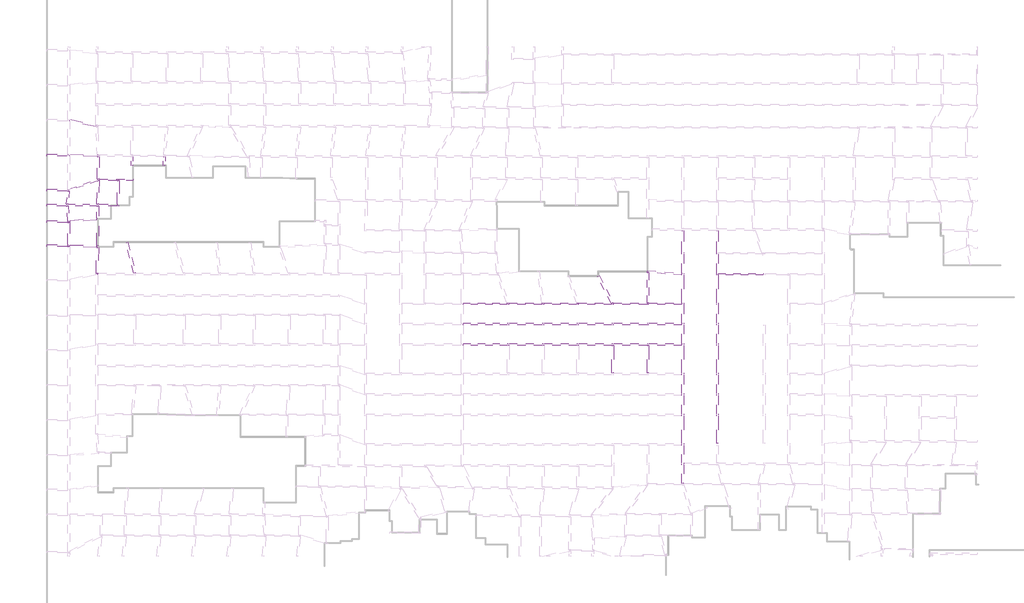
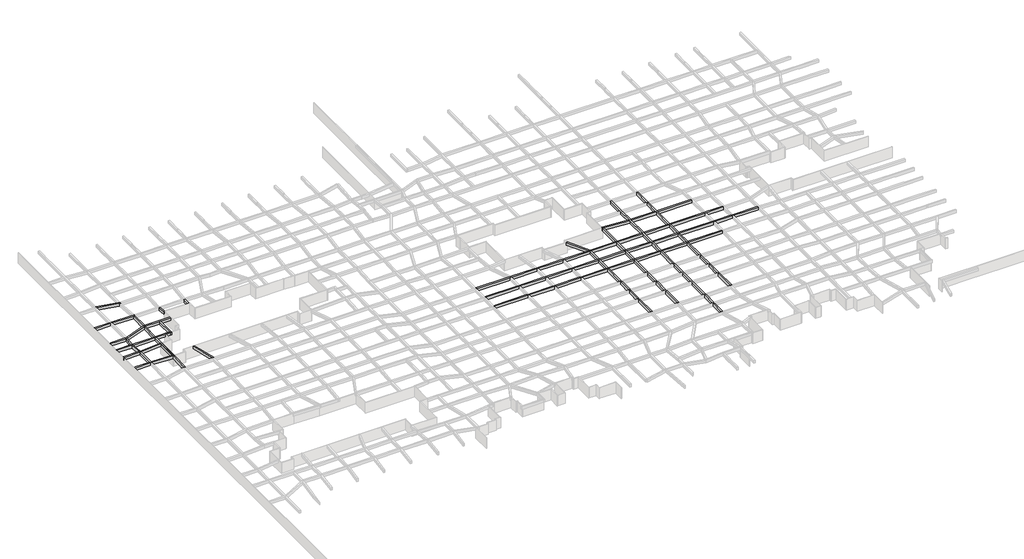
# One storey, part 34 of 45: 33 beams.
"""IFC4 building model written with IfcOpenShell, lengths in millimetres."""

import ifcopenshell
import ifcopenshell.guid

model = None  # the IFC model being written
_history = None  # IfcOwnerHistory: only IFC2X3 demands one
_inside = {}  # id of a spatial element -> (the spatial element, [elements in it])
_under = {}  # id of a project, library or spatial element -> (it, [spatial elements below it])
_declared = {}  # id of a project -> (the project, [libraries it declares])
_typed = {}  # id of a type object -> (the type object, [elements of that type])
_made_of = {}  # id of a material, layer set ... -> (it, [elements and type objects made of it])


def new_model(schema):
    """Start an empty IFC model of exactly this schema.

    Asked for "IFC4X3", IfcOpenShell would pick the latest addendum, in which some entities
    have other attributes; the version numbers below select the first issue.
    IFC2X3 requires an IfcOwnerHistory on every rooted entity: one is made here for all.
    """
    global model, _history
    if schema == "IFC4X3":
        model = ifcopenshell.file(schema_version=(4, 3, 0, 0))
    else:
        model = ifcopenshell.file(schema=schema)
    _inside.clear()
    _under.clear()
    _declared.clear()
    _typed.clear()
    _made_of.clear()
    _history = None
    if model.schema == "IFC2X3":
        org = make("IfcOrganization", Name="unknown")
        user = make(
            "IfcPersonAndOrganization",
            ThePerson=make("IfcPerson", FamilyName="unknown"),
            TheOrganization=org,
        )
        app = make(
            "IfcApplication",
            ApplicationDeveloper=org,
            Version="unknown",
            ApplicationFullName="unknown",
            ApplicationIdentifier="unknown",
        )
        _history = make(
            "IfcOwnerHistory",
            OwningUser=user,
            OwningApplication=app,
            ChangeAction="ADDED",
            CreationDate=0,
        )
    return model


def make(cls, **values):
    """One entity of the class cls with the attributes given. An attribute that is None is left unset."""
    return model.create_entity(
        cls, **{name: value for name, value in values.items() if value is not None}
    )


def rooted(cls, **values):
    """An entity with a GlobalId (a new one), such as an element, a storey or a relation."""
    return make(cls, GlobalId=ifcopenshell.guid.new(), OwnerHistory=_history, **values)


def si_unit(unit_type, name, prefix=None):
    """IfcSIUnit, for example si_unit("LENGTHUNIT", "METRE", prefix="MILLI")."""
    return make("IfcSIUnit", UnitType=unit_type, Prefix=prefix, Name=name)


def assignment(units):
    """IfcUnitAssignment: the units of a project."""
    return None if units is None else make("IfcUnitAssignment", Units=units)


def point(xyz):
    """IfcCartesianPoint."""
    return None if xyz is None else make("IfcCartesianPoint", Coordinates=xyz)


def direction(xyz):
    """IfcDirection."""
    return None if xyz is None else make("IfcDirection", DirectionRatios=xyz)


def frame(location, z_axis=None, x_axis=None):
    """IfcAxis2Placement3D, a coordinate frame: its origin and axes. An axis left out is left unset."""
    return make(
        "IfcAxis2Placement3D",
        Location=point(location),
        Axis=direction(z_axis),
        RefDirection=direction(x_axis),
    )


def origin():
    """The frame at (0, 0, 0) with its axes left unset."""
    return frame((0.0, 0.0, 0.0))


def place(relative_to, where):
    """IfcLocalPlacement: puts the frame where relative to a parent placement (None: the world)."""
    return make(
        "IfcLocalPlacement", PlacementRelTo=relative_to, RelativePlacement=where
    )


def context(
    kind, dimensions, precision=None, world=None, true_north=None, identifier=None
):
    """IfcGeometricRepresentationContext, for example the 3D "Model" context."""
    return make(
        "IfcGeometricRepresentationContext",
        ContextIdentifier=identifier,
        ContextType=kind,
        CoordinateSpaceDimension=dimensions,
        Precision=precision,
        WorldCoordinateSystem=world,
        TrueNorth=true_north,
    )


def project(units=None, contexts=None):
    """IfcProject with its units and contexts."""
    return rooted(
        "IfcProject",
        Name="project",
        RepresentationContexts=contexts,
        UnitsInContext=assignment(units),
    )


def spatial(cls, under=None, at=None, **own):
    """A site, building, storey or space (cls), placed at a placement, below another one or the project."""
    s = rooted(cls, ObjectPlacement=at, **own)
    if under is not None:
        _under.setdefault(under.id(), (under, []))[1].append(s)
    return s


def polyline(points):
    """IfcPolyline through the points."""
    return make("IfcPolyline", Points=[point(p) for p in points])


def outline(outer, holes=None, kind="AREA"):
    """IfcArbitraryClosedProfileDef: a profile drawn as a closed curve; with holes, ...WithVoids."""
    if holes is None:
        return make("IfcArbitraryClosedProfileDef", ProfileType=kind, OuterCurve=outer)
    return make(
        "IfcArbitraryProfileDefWithVoids",
        ProfileType=kind,
        OuterCurve=outer,
        InnerCurves=holes,
    )


def extrude(swept, where, along, depth):
    """IfcExtrudedAreaSolid: the profile swept, set in the frame where, extruded along a direction by depth."""
    return make(
        "IfcExtrudedAreaSolid",
        SweptArea=swept,
        Position=where,
        ExtrudedDirection=direction(along),
        Depth=depth,
    )


def faces_of(points, faces, orient=None, outer=None):
    """IfcFace entities. A face is a list of loops; a loop is a list of indices into points, from 0.

    orient and outer hold one flag for each loop. By default every Orientation is true, the
    first loop of a face is its IfcFaceOuterBound and the others are IfcFaceBound.
    """
    made = []
    for i, loops in enumerate(faces):
        bounds = []
        for j, loop in enumerate(loops):
            is_outer = j == 0 if outer is None else outer[i][j]
            bounds.append(
                make(
                    "IfcFaceOuterBound" if is_outer else "IfcFaceBound",
                    Bound=make("IfcPolyLoop", Polygon=[points[k] for k in loop]),
                    Orientation=True if orient is None else orient[i][j],
                )
            )
        made.append(make("IfcFace", Bounds=bounds))
    return made


def faceted_brep(points, faces, orient=None, outer=None, voids=None):
    """IfcFacetedBrep: a solid bounded by flat faces; with voids (closed shells), ...WithVoids."""
    shared = [point(p) for p in points]
    hull = make("IfcClosedShell", CfsFaces=faces_of(shared, faces, orient, outer))
    if voids is None:
        return make("IfcFacetedBrep", Outer=hull)
    return make(
        "IfcFacetedBrepWithVoids",
        Outer=hull,
        Voids=[
            make(cls, CfsFaces=faces_of(shared, fs, o, b)) for cls, fs, o, b in voids
        ],
    )


def shape(context_of_items, identifier, shape_type, items):
    """IfcShapeRepresentation: the items that make up one representation, for example the "Body"."""
    return make(
        "IfcShapeRepresentation",
        ContextOfItems=context_of_items,
        RepresentationIdentifier=identifier,
        RepresentationType=shape_type,
        Items=items,
    )


def made_of(thing, what):
    """Note that an element or type object is made of a material, layer set ...; save() writes the relation."""
    if what is not None:
        _made_of.setdefault(what.id(), (what, []))[1].append(thing)
    return thing


def element(
    cls,
    number,
    at=None,
    inside=None,
    cuts=None,
    type_object=None,
    material=None,
    context=None,
    identifier="Body",
    shape_type=None,
    held_by="IfcProductDefinitionShape",
    body=None,
    shapes=None,
    **own,
):
    """One element of the class cls, such as IfcWall. Its Tag is "e" and its number.

    at: its placement. inside: the storey or other place that contains it. cuts: it is an
    opening in that element (IfcRelVoidsElement). A single representation is given by context,
    identifier, shape_type and body (its items); several are given by shapes. held_by: the class
    of the entity that holds the representations. save() writes the other relations.
    """
    e = rooted(cls, Tag="e%d" % number, ObjectPlacement=at, **own)
    if body is not None:
        shapes = [shape(context, identifier, shape_type, body)]
    if shapes is not None:
        e.Representation = make(held_by, Representations=shapes)
    if inside is not None:
        _inside.setdefault(inside.id(), (inside, []))[1].append(e)
    if cuts is not None:
        rooted(
            "IfcRelVoidsElement", RelatingBuildingElement=cuts, RelatedOpeningElement=e
        )
    if type_object is not None:
        _typed.setdefault(type_object.id(), (type_object, []))[1].append(e)
    return made_of(e, material)


def aggregate(whole, parts):
    """IfcRelAggregates: a whole, such as a stair, and the parts it consists of."""
    return rooted("IfcRelAggregates", RelatingObject=whole, RelatedObjects=parts)


def save(model, path):
    """Write the relations noted so far, then the file.

    IfcRelAggregates (storeys below a building ...), IfcRelContainedInSpatialStructure (elements
    in a storey), IfcRelDefinesByType, IfcRelAssociatesMaterial and IfcRelDeclares: one each for
    every whole, place, type object, material and project.
    """
    for whole, parts in _under.values():
        aggregate(whole, parts)
    for where, things in _inside.values():
        rooted(
            "IfcRelContainedInSpatialStructure",
            RelatedElements=things,
            RelatingStructure=where,
        )
    for kind, things in _typed.values():
        rooted("IfcRelDefinesByType", RelatedObjects=things, RelatingType=kind)
    for what, things in _made_of.values():
        rooted("IfcRelAssociatesMaterial", RelatedObjects=things, RelatingMaterial=what)
    for by, libraries in _declared.values():
        rooted("IfcRelDeclares", RelatingContext=by, RelatedDefinitions=libraries)
    model.write(path)


model = new_model("IFC4")

# Units and contexts
model_context = context("Model", 3, world=origin())
ifc_project = project(units=[si_unit("LENGTHUNIT", "METRE", prefix="MILLI")], contexts=[model_context])

# Site, building, storey
site = spatial("IfcSite", under=ifc_project)
building = spatial("IfcBuilding", under=site)
storey = spatial("IfcBuildingStorey", under=building, Name="户型图", Elevation=0.0)

# Beams
placement = place(None, origin())
element("IfcBeam", 1, ObjectType="混凝土 - 矩形梁 : KL_beam", at=placement, inside=storey, context=model_context, shape_type="Brep", body=[
    faceted_brep([(-143382.0266166, 146959.1608501, 3300.0), (-143382.0266166, 147100.0740901, 3300.0), (-143382.0266166, 147301.8194636, 3300.0), (-143382.0266166, 147382.2091225, 3300.0), (-143782.0266166, 147244.4780772, 3300.0), (-149980.0650049, 145110.3223119, 3300.0), (-149980.0650049, 144687.2740394, 3300.0), (-143786.9810795, 146819.7238463, 3300.0), (-143384.5011388, 146958.3088037, 3300.0), (-143382.0266166, 146959.1608501, 2500.0), (-149980.0650049, 144687.2740394, 2500.0), (-143786.9810795, 146819.7238463, 2500.0), (-143384.5011388, 146958.3088037, 2500.0), (-143382.0266166, 147382.2091225, 2500.0), (-143382.0266166, 147301.8194636, 2500.0), (-143382.0266166, 147100.0740901, 2500.0), (-149980.0650049, 145110.3223119, 2500.0), (-143782.0266166, 147244.4780772, 2500.0)], [[[0, 1, 2, 3, 4, 5, 6, 7, 8]], [[9, 0, 8, 7, 6, 10, 11, 12]], [[13, 14, 15, 9, 12, 11, 10, 16, 17]], [[3, 13, 17, 16, 5, 4]], [[6, 5, 16, 10]], [[3, 2, 1, 0, 9, 15, 14, 13]]]),
])
element("IfcBeam", 2, ObjectType="混凝土 - 矩形梁 : KL_beam", at=placement, inside=storey, context=model_context, shape_type="SweptSolid", body=[
    extrude(outline(polyline([(-155040.2933307, 152429.932653), (-155040.2933307, 152829.932653), (-150380.0650049, 152829.932653), (-150380.0650049, 152429.932653), (-155040.2933307, 152429.932653)])), frame((0.0, 0.0, 2500.0), z_axis=(0.0, 0.0, 1.0), x_axis=(1.0, 0.0, 0.0)), (0.0, 0.0, 1.0), 800.0),
])
element("IfcBeam", 3, ObjectType="混凝土 - 矩形梁 : KL_beam", at=placement, inside=storey, context=model_context, shape_type="Brep", body=[
    faceted_brep([(-155040.2933307, 145029.932653, 3300.0), (-155040.2933307, 145029.932653, 2500.0), (-155040.2933307, 144629.932653, 2500.0), (-155040.2933307, 144629.932653, 3300.0), (-150398.2249808, 144629.932653, 3300.0), (-150146.5964831, 144629.932653, 3300.0), (-149992.0411016, 144683.1503386, 3300.0), (-149980.0650049, 144687.2740394, 3300.0), (-150380.0650049, 144687.2740394, 3300.0), (-150380.0650049, 144972.5912666, 3300.0), (-150380.0650049, 145029.932653, 3300.0), (-150398.2249808, 144629.932653, 2500.0), (-150146.5964831, 144629.932653, 2500.0), (-150380.0650049, 145029.932653, 2500.0), (-150380.0650049, 144972.5912666, 2500.0), (-150380.0650049, 144687.2740394, 2500.0), (-149980.0650049, 144687.2740394, 2500.0), (-149992.0411016, 144683.1503386, 2500.0)], [[[0, 1, 2, 3]], [[0, 3, 4, 5, 6, 7, 8, 9, 10]], [[3, 2, 11, 12, 5, 4]], [[2, 1, 13, 14, 15, 16, 17, 12, 11]], [[1, 0, 10, 13]], [[7, 6, 5, 12, 17, 16]], [[8, 15, 14, 13, 10, 9]], [[15, 8, 7, 16]]]),
])
element("IfcBeam", 4, ObjectType="混凝土 - 矩形梁 : KL_beam", at=placement, inside=storey, context=model_context, shape_type="Brep", body=[
    faceted_brep([(-143707.512981, 158849.6325984, 3300.0), (-143710.0525927, 158899.3775215, 3300.0), (-143728.6193094, 159263.055125, 3300.0), (-143899.5027499, 159299.3775215, 3300.0), (-144130.8224936, 159348.5460509, 3300.0), (-149980.0650049, 160591.8409275, 3300.0), (-149980.0650049, 160182.9046895, 3300.0), (-144112.4278844, 158935.6999181, 3300.0), (-143707.512981, 158849.6325984, 2500.0), (-149980.0650049, 160182.9046895, 2500.0), (-144112.4278844, 158935.6999181, 2500.0), (-143728.6193094, 159263.055125, 2500.0), (-143710.0525927, 158899.3775215, 2500.0), (-149980.0650049, 160591.8409275, 2500.0), (-144130.8224936, 159348.5460509, 2500.0), (-143899.5027499, 159299.3775215, 2500.0)], [[[0, 1, 2, 3, 4, 5, 6, 7]], [[8, 0, 7, 6, 9, 10]], [[11, 12, 8, 10, 9, 13, 14, 15]], [[2, 11, 15, 14, 13, 5, 4, 3]], [[6, 5, 13, 9]], [[2, 1, 0, 8, 12, 11]]]),
])
element("IfcBeam", 5, ObjectType="混凝土 - 矩形梁 : KL_beam", at=placement, inside=storey, context=model_context, shape_type="Brep", body=[
    faceted_brep([(-143401.4944506, 152264.5687631, 3300.0), (-143391.7428195, 152664.4498776, 3300.0), (-143792.7630206, 152674.2292868, 3300.0), (-149980.0650049, 152825.1148483, 3300.0), (-149980.0650049, 152424.9959274, 3300.0), (-143782.0266166, 152273.8485445, 3300.0), (-143401.4944506, 152264.5687631, 2500.0), (-149980.0650049, 152424.9959274, 2500.0), (-143782.0266166, 152273.8485445, 2500.0), (-143391.7428195, 152664.4498776, 2500.0), (-149980.0650049, 152825.1148483, 2500.0), (-143792.7630206, 152674.2292868, 2500.0)], [[[0, 1, 2, 3, 4, 5]], [[6, 0, 5, 4, 7, 8]], [[9, 6, 8, 7, 10, 11]], [[1, 9, 11, 10, 3, 2]], [[4, 3, 10, 7]], [[1, 0, 6, 9]]]),
])
element("IfcBeam", 6, ObjectType="混凝土 - 矩形梁 : KL_beam", at=placement, inside=storey, context=model_context, shape_type="Brep", body=[
    faceted_brep([(-143382.0266166, 147382.2091225, 3300.0), (-143382.0266166, 152269.0307398, 3300.0), (-143382.0266166, 152664.2129351, 3300.0), (-143391.7428195, 152664.4498776, 3300.0), (-143401.4944506, 152264.5687631, 3300.0), (-143772.3104136, 152273.611602, 3300.0), (-143782.0266166, 152273.8485445, 3300.0), (-143782.0266166, 147244.4780772, 3300.0), (-143782.0266166, 147244.4780772, 2500.0), (-143782.0266166, 152273.8485445, 2500.0), (-143382.0266166, 152664.2129351, 2500.0), (-143382.0266166, 152269.0307398, 2500.0), (-143382.0266166, 147382.2091225, 2500.0), (-143772.3104136, 152273.611602, 2500.0), (-143401.4944506, 152264.5687631, 2500.0), (-143391.7428195, 152664.4498776, 2500.0)], [[[0, 1, 2, 3, 4, 5, 6, 7]], [[8, 7, 6, 9]], [[10, 11, 12, 8, 9, 13, 14, 15]], [[2, 1, 0, 12, 11, 10]], [[15, 3, 2, 10]], [[0, 7, 8, 12]], [[4, 14, 13, 9, 6, 5]], [[14, 4, 3, 15]]]),
])
element("IfcBeam", 7, ObjectType="混凝土 - 矩形梁 : KL_beam", at=placement, inside=storey, context=model_context, shape_type="Brep", body=[
    faceted_brep([(-143384.5011388, 146958.3088037, 3300.0), (-143782.0266166, 146821.4298047, 3300.0), (-143786.9810795, 146819.7238463, 3300.0), (-143876.8568673, 141670.7434089, 3300.0), (-143476.7959361, 141670.7434089, 3300.0), (-143385.4871639, 146901.8194636, 3300.0), (-143786.9810795, 146819.7238463, 2500.0), (-143876.8568673, 141670.7434089, 2500.0), (-143782.0266166, 146821.4298047, 2500.0), (-143384.5011388, 146958.3088037, 2500.0), (-143385.4871639, 146901.8194636, 2500.0), (-143476.7959361, 141670.7434089, 2500.0)], [[[0, 1, 2, 3, 4, 5]], [[2, 6, 7, 3]], [[6, 8, 9, 10, 11, 7]], [[9, 0, 5, 4, 11, 10]], [[6, 2, 1, 0, 9, 8]], [[4, 3, 7, 11]]]),
    faceted_brep([(-143378.505138, 147301.8194636, 3300.0), (-143378.505138, 147301.8194636, 2500.0), (-143382.0266166, 147301.8194636, 2500.0), (-143382.0266166, 147301.8194636, 3300.0), (-143382.0266166, 147100.0740901, 3300.0), (-143382.0266166, 147100.0740901, 2500.0)], [[[0, 1, 2, 3]], [[4, 3, 2, 5]], [[3, 4, 0]], [[5, 2, 1]], [[1, 0, 4, 5]]]),
])
element("IfcBeam", 8, ObjectType="混凝土 - 矩形梁 : KL_beam", at=placement, inside=storey, context=model_context, shape_type="Brep", body=[
    faceted_brep([(-135832.9708868, 147301.8194636, 3300.0), (-135832.9708868, 146901.8194636, 3300.0), (-135832.9708868, 146901.8194636, 2500.0), (-135832.9708868, 147301.8194636, 2500.0), (-143378.505138, 147301.8194636, 3300.0), (-143382.0266166, 147100.0740901, 3300.0), (-143382.0266166, 146959.1608501, 3300.0), (-143384.5011388, 146958.3088037, 3300.0), (-143385.4871639, 146901.8194636, 3300.0), (-139332.9151571, 146901.8194636, 3300.0), (-138932.9151571, 146901.8194636, 3300.0), (-143385.4871639, 146901.8194636, 2500.0), (-139332.9151571, 146901.8194636, 2500.0), (-138932.9151571, 146901.8194636, 2500.0), (-143384.5011388, 146958.3088037, 2500.0), (-143382.0266166, 146959.1608501, 2500.0), (-143382.0266166, 147100.0740901, 2500.0), (-143378.505138, 147301.8194636, 2500.0)], [[[0, 1, 2, 3]], [[1, 0, 4, 5, 6, 7, 8, 9, 10]], [[2, 1, 10, 9, 8, 11, 12, 13]], [[3, 2, 13, 12, 11, 14, 15, 16, 17]], [[0, 3, 17, 4]], [[6, 15, 14, 7]], [[15, 6, 5, 16]], [[8, 7, 14, 11]], [[5, 4, 17, 16]]]),
])
element("IfcBeam", 9, ObjectType="混凝土 - 矩形梁 : KL_beam", at=placement, inside=storey, context=model_context, shape_type="SweptSolid", body=[
    extrude(outline(polyline([(-135785.0673191, 150256.2984935), (-136183.5451983, 150221.4361964), (-136359.3151276, 152230.4956807), (-135957.7871926, 152230.4956807), (-135785.0673191, 150256.2984935)])), frame((0.0, 0.0, 2500.0), z_axis=(0.0, 0.0, 1.0), x_axis=(1.0, 0.0, 0.0)), (0.0, 0.0, 1.0), 800.0),
])
element("IfcBeam", 10, ObjectType="混凝土 - 矩形梁 : KL_beam", at=placement, inside=storey, context=model_context, shape_type="SweptSolid", body=[
    extrude(outline(polyline([(-128664.001285, 150230.335265), (-129064.001285, 150230.335265), (-129064.001285, 152230.4956807), (-128664.001285, 152230.4956807), (-128664.001285, 150230.335265)])), frame((0.0, 0.0, 2500.0), z_axis=(0.0, 0.0, 1.0), x_axis=(1.0, 0.0, 0.0)), (0.0, 0.0, 1.0), 800.0),
])
element("IfcBeam", 11, ObjectType="混凝土 - 矩形梁 : KL_beam", at=placement, inside=storey, context=model_context, shape_type="SweptSolid", body=[
    extrude(outline(polyline([(-150398.2249808, 144629.932653), (-150146.5964831, 144629.932653), (-149992.0411016, 144683.1503386), (-150255.5925579, 141670.7434089), (-150657.1204929, 141670.7434089), (-150398.2249808, 144629.932653)])), frame((0.0, 0.0, 2500.0), z_axis=(0.0, 0.0, 1.0), x_axis=(1.0, 0.0, 0.0)), (0.0, 0.0, 1.0), 800.0),
])
element("IfcBeam", 12, ObjectType="混凝土 - 矩形梁 : KL_beam", at=placement, inside=storey, context=model_context, shape_type="Brep", body=[
    faceted_brep([(-150343.4616022, 137629.932653, 3300.0), (-149944.983723, 137664.7949501, 3300.0), (-149978.3875763, 138046.6027411, 3300.0), (-150260.4633344, 141270.7434089, 3300.0), (-150661.9912694, 141270.7434089, 3300.0), (-150378.4570676, 138029.932653, 3300.0), (-150343.4616022, 137629.932653, 2500.0), (-150661.9912694, 141270.7434089, 2500.0), (-150378.4570676, 138029.932653, 2500.0), (-149944.983723, 137664.7949501, 2500.0), (-150260.4633344, 141270.7434089, 2500.0), (-149978.3875763, 138046.6027411, 2500.0)], [[[0, 1, 2, 3, 4, 5]], [[6, 0, 5, 4, 7, 8]], [[9, 6, 8, 7, 10, 11]], [[1, 9, 11, 10, 3, 2]], [[1, 0, 6, 9]], [[3, 10, 7, 4]]]),
])
element("IfcBeam", 13, ObjectType="混凝土 - 矩形梁 : KL_beam", at=placement, inside=storey, context=model_context, shape_type="Brep", body=[
    faceted_brep([(-155040.3585119, 138029.932653, 3300.0), (-155040.3585119, 138029.932653, 2500.0), (-155040.3585119, 137629.932653, 2500.0), (-155040.3585119, 137629.932653, 3300.0), (-150359.8528414, 137629.932653, 3300.0), (-150343.4616022, 137629.932653, 3300.0), (-150378.4570676, 138029.932653, 3300.0), (-150359.8528414, 137629.932653, 2500.0), (-150343.4616022, 137629.932653, 2500.0), (-150378.4570676, 138029.932653, 2500.0)], [[[0, 1, 2, 3]], [[0, 3, 4, 5, 6]], [[3, 2, 7, 8, 5, 4]], [[2, 1, 9, 8, 7]], [[1, 0, 6, 9]], [[6, 5, 8, 9]]]),
])
element("IfcBeam", 14, ObjectType="混凝土 - 矩形梁 : KL_beam", at=placement, inside=storey, context=model_context, shape_type="Brep", body=[
    faceted_brep([(-150343.4616022, 137629.932653, 3300.0), (-150151.4631788, 137629.932653, 3300.0), (-149959.8528414, 137646.6963853, 3300.0), (-143879.7600926, 138178.635574, 3300.0), (-143879.7600926, 138580.163509, 3300.0), (-149978.3875763, 138046.6027411, 3300.0), (-149944.983723, 137664.7949501, 3300.0), (-150151.4631788, 137629.932653, 2500.0), (-149959.8528414, 137646.6963853, 2500.0), (-143879.7600926, 138178.635574, 2500.0), (-150343.4616022, 137629.932653, 2500.0), (-149944.983723, 137664.7949501, 2500.0), (-149978.3875763, 138046.6027411, 2500.0), (-143879.7600926, 138580.163509, 2500.0)], [[[0, 1, 2, 3, 4, 5, 6]], [[1, 7, 8, 9, 3, 2]], [[7, 10, 11, 12, 13, 9, 8]], [[12, 5, 4, 13]], [[1, 0, 10, 7]], [[11, 6, 5, 12]], [[6, 11, 10, 0]], [[4, 3, 9, 13]]]),
])
element("IfcBeam", 15, ObjectType="混凝土 - 矩形梁 : KL_beam", at=placement, inside=storey, context=model_context, shape_type="Brep", body=[
    faceted_brep([(-149959.8528414, 137646.6963853, 3300.0), (-150151.4631788, 137629.932653, 3300.0), (-150343.4616022, 137629.932653, 3300.0), (-150359.8528414, 137629.932653, 3300.0), (-150359.8528414, 132629.932653, 3300.0), (-150359.8528414, 132236.8248652, 3300.0), (-150162.4857077, 132229.932653, 3300.0), (-149959.8528414, 132222.8565574, 3300.0), (-149959.8528414, 132623.1003751, 3300.0), (-150359.8528414, 132236.8248652, 2500.0), (-150359.8528414, 137629.932653, 2500.0), (-150359.8528414, 132629.932653, 2500.0), (-150343.4616022, 137629.932653, 2500.0), (-150151.4631788, 137629.932653, 2500.0), (-149959.8528414, 137646.6963853, 2500.0), (-149959.8528414, 132623.1003751, 2500.0), (-149959.8528414, 132222.8565574, 2500.0), (-150162.4857077, 132229.932653, 2500.0)], [[[0, 1, 2, 3, 4, 5, 6, 7, 8]], [[9, 5, 4, 3, 10, 11]], [[10, 12, 13, 14, 15, 16, 17, 9, 11]], [[14, 0, 8, 7, 16, 15]], [[13, 1, 0, 14]], [[1, 13, 12, 10, 3, 2]], [[7, 6, 5, 9, 17, 16]]]),
])
element("IfcBeam", 16, ObjectType="混凝土 - 矩形梁 : KL_beam", at=placement, inside=storey, context=model_context, shape_type="Brep", body=[
    faceted_brep([(-143484.3485413, 131996.7269644, 3300.0), (-143479.7600926, 132128.122943, 3300.0), (-143479.7600926, 132186.4660021, 3300.0), (-143486.3834443, 131996.7980247, 3300.0), (-143484.3485413, 131996.7269644, 2500.0), (-143486.3834443, 131996.7980247, 2500.0), (-143479.7600926, 132128.122943, 2500.0), (-143479.7600926, 132186.4660021, 2500.0)], [[[0, 1, 2, 3]], [[4, 0, 3, 5]], [[6, 4, 5, 7]], [[0, 4, 6, 1]], [[1, 6, 7, 2]], [[3, 2, 7, 5]]]),
    faceted_brep([(-149959.8528414, 132623.1003751, 2500.0), (-149959.8528414, 132623.1003751, 3300.0), (-143879.7600926, 132410.7788577, 3300.0), (-143879.7600926, 132410.7788577, 2500.0), (-149959.8528414, 132222.8565574, 3300.0), (-149959.8528414, 132222.8565574, 2500.0), (-143879.7600926, 132193.4480281, 3300.0), (-143879.7600926, 132010.53504, 3300.0), (-143879.7600926, 132010.53504, 2500.0), (-143879.7600926, 132193.4480281, 2500.0), (-143886.1397751, 132010.7578234, 3300.0), (-143886.1397751, 132010.7578234, 2500.0)], [[[0, 1, 2, 3]], [[4, 1, 0, 5]], [[2, 6, 7, 8, 9, 3]], [[1, 4, 10, 7, 6, 2]], [[4, 5, 11, 8, 7, 10]], [[5, 0, 3, 9, 8, 11]]]),
])
element("IfcBeam", 17, ObjectType="混凝土 - 矩形梁 : KL_beam", at=placement, inside=storey, context=model_context, shape_type="Brep", body=[
    faceted_brep([(-155040.2581756, 132629.932653, 3300.0), (-155040.2581756, 132629.932653, 2500.0), (-155040.2581756, 132229.932653, 2500.0), (-155040.2581756, 132229.932653, 3300.0), (-150359.8528414, 132229.932653, 2500.0), (-150162.4857077, 132229.932653, 2500.0), (-150162.4857077, 132229.932653, 3300.0), (-150359.8528414, 132229.932653, 3300.0), (-150359.8528414, 132236.8248652, 2500.0), (-150359.8528414, 132236.8248652, 3300.0), (-150359.8528414, 132629.932653, 2500.0), (-150359.8528414, 132629.932653, 3300.0)], [[[0, 1, 2, 3]], [[3, 2, 4, 5, 6, 7]], [[8, 9, 6, 5]], [[9, 8, 10, 11]], [[0, 3, 7, 6, 9, 11]], [[2, 1, 10, 8, 5, 4]], [[1, 0, 11, 10]]]),
])
element("IfcBeam", 18, ObjectType="混凝土 - 矩形梁 : KL_beam", at=placement, inside=storey, context=model_context, shape_type="Brep", body=[
    faceted_brep([(-143879.7600926, 132193.4480281, 3300.0), (-143872.1799765, 132410.5141542, 3300.0), (-143479.7600926, 132396.8105499, 3300.0), (-143479.7600926, 141270.7434089, 3300.0), (-143879.7600926, 141270.7434089, 3300.0), (-143879.7600926, 138580.163509, 3300.0), (-143879.7600926, 138178.635574, 3300.0), (-143879.7600926, 132410.7788577, 3300.0), (-143879.7600926, 132193.4480281, 2500.0), (-143879.7600926, 141270.7434089, 2500.0), (-143879.7600926, 138580.163509, 2500.0), (-143879.7600926, 138178.635574, 2500.0), (-143879.7600926, 132410.7788577, 2500.0), (-143872.1799765, 132410.5141542, 2500.0), (-143479.7600926, 141270.7434089, 2500.0), (-143479.7600926, 132396.8105499, 2500.0)], [[[0, 1, 2, 3, 4, 5, 6, 7]], [[8, 0, 7, 6, 5, 4, 9, 10, 11, 12]], [[13, 8, 12, 11, 10, 9, 14, 15]], [[2, 15, 14, 3]], [[13, 1, 0, 8]], [[1, 13, 15, 2]], [[3, 14, 9, 4]]]),
])
element("IfcBeam", 19, ObjectType="混凝土 - 矩形梁 : KL_beam", at=placement, inside=storey, context=model_context, shape_type="Brep", body=[
    faceted_brep([(-143695.7753192, 126000.5992612, 2500.0), (-143695.7753192, 126000.5992612, 3300.0), (-143733.590805, 126001.9198071, 3300.0), (-143733.590805, 126001.9198071, 2500.0), (-143685.6713407, 126289.9393475, 3300.0), (-143486.3834443, 131996.7980247, 3300.0), (-143879.7600926, 132010.53504, 3300.0), (-143886.1397751, 132010.7578234, 3300.0), (-144086.9200457, 126261.1631403, 3300.0), (-144087.2760394, 126250.9688143, 3300.0), (-143733.590805, 126250.9688143, 3300.0), (-143886.1397751, 132010.7578234, 2500.0), (-144086.9200457, 126261.1631403, 2500.0), (-144087.2760394, 126250.9688143, 2500.0), (-143486.3834443, 131996.7980247, 2500.0), (-143685.6713407, 126289.9393475, 2500.0), (-143733.590805, 126250.9688143, 2500.0), (-143879.7600926, 132010.53504, 2500.0)], [[[0, 1, 2, 3]], [[1, 4, 5, 6, 7, 8, 9, 10, 2]], [[7, 11, 12, 13, 9, 8]], [[14, 15, 0, 3, 16, 13, 12, 11, 17]], [[1, 0, 15, 14, 5, 4]], [[7, 6, 5, 14, 17, 11]], [[10, 16, 3, 2]], [[16, 10, 9, 13]]]),
])
element("IfcBeam", 20, ObjectType="混凝土 - 矩形梁 : KL_beam", at=placement, inside=storey, context=model_context, shape_type="SweptSolid", body=[
    extrude(outline(polyline([(-137393.6797881, 133124.7137702), (-137005.5614976, 133221.4825284), (-135277.3336797, 126289.9393475), (-135689.5791314, 126289.9393475), (-137393.6797881, 133124.7137702)])), frame((0.0, 0.0, 2500.0), z_axis=(0.0, 0.0, 1.0), x_axis=(1.0, 0.0, 0.0)), (0.0, 0.0, 1.0), 800.0),
])
element("IfcBeam", 21, ObjectType="混凝土 - 矩形梁 : KL_beam", at=placement, inside=storey, context=model_context, shape_type="Brep", body=[
    faceted_brep([(-139332.9151571, 141270.7434089, 3300.0), (-138932.9151571, 141270.7434089, 3300.0), (-138932.9151571, 146901.8194636, 3300.0), (-139332.9151571, 146901.8194636, 3300.0), (-139332.9151571, 141670.7434089, 3300.0), (-138932.9151571, 141270.7434089, 2500.0), (-138932.9151571, 146901.8194636, 2500.0), (-139332.9151571, 141270.7434089, 2500.0), (-139332.9151571, 141670.7434089, 2500.0), (-139332.9151571, 146901.8194636, 2500.0)], [[[0, 1, 2, 3, 4]], [[1, 5, 6, 2]], [[5, 7, 8, 9, 6]], [[7, 0, 4, 3, 9, 8]], [[3, 2, 6, 9]], [[1, 0, 7, 5]]]),
])
element("IfcBeam", 22, ObjectType="混凝土 - 矩形梁 : KL_beam", at=placement, inside=storey, context=model_context, shape_type="Brep", body=[
    faceted_brep([(-155040.2184067, 141270.7434089, 3300.0), (-155040.2184067, 141670.7434089, 3300.0), (-155040.2184067, 141670.7434089, 2500.0), (-155040.2184067, 141270.7434089, 2500.0), (-150661.9912694, 141270.7434089, 3300.0), (-150260.4633344, 141270.7434089, 3300.0), (-143879.7600926, 141270.7434089, 3300.0), (-143479.7600926, 141270.7434089, 3300.0), (-139332.9151571, 141270.7434089, 3300.0), (-139332.9151571, 141670.7434089, 3300.0), (-143476.7959361, 141670.7434089, 3300.0), (-143876.8568673, 141670.7434089, 3300.0), (-150255.5925579, 141670.7434089, 3300.0), (-150657.1204929, 141670.7434089, 3300.0), (-139332.9151571, 141670.7434089, 2500.0), (-143476.7959361, 141670.7434089, 2500.0), (-143876.8568673, 141670.7434089, 2500.0), (-150255.5925579, 141670.7434089, 2500.0), (-150657.1204929, 141670.7434089, 2500.0), (-139332.9151571, 141270.7434089, 2500.0), (-143479.7600926, 141270.7434089, 2500.0), (-143879.7600926, 141270.7434089, 2500.0), (-150260.4633344, 141270.7434089, 2500.0), (-150661.9912694, 141270.7434089, 2500.0)], [[[0, 1, 2, 3]], [[1, 0, 4, 5, 6, 7, 8, 9, 10, 11, 12, 13]], [[2, 1, 13, 12, 11, 10, 9, 14, 15, 16, 17, 18]], [[3, 2, 18, 17, 16, 15, 14, 19, 20, 21, 22, 23]], [[0, 3, 23, 22, 21, 20, 19, 8, 7, 6, 5, 4]], [[9, 8, 19, 14]]]),
])
element("IfcBeam", 23, ObjectType="混凝土 - 矩形梁 : KL_beam", at=placement, inside=storey, context=model_context, shape_type="Brep", body=[
    faceted_brep([(-13220.6748317, 135822.9605472, 3300.0), (-13620.6748317, 135822.9605472, 3300.0), (-13620.6748317, 130936.5288825, 3300.0), (-13620.6748317, 130536.5288825, 3300.0), (-13620.6748317, 126278.4896927, 3300.0), (-13620.6748317, 125877.3143948, 3300.0), (-13620.6748317, 119662.5591329, 3300.0), (-13620.6748317, 119262.5591329, 3300.0), (-13620.6748317, 115171.853595, 3300.0), (-13620.6748317, 114771.853595, 3300.0), (-13620.6748317, 110629.932653, 3300.0), (-13620.6748317, 110229.932653, 3300.0), (-13620.6748317, 104011.2459144, 3300.0), (-13620.6748317, 103611.2459144, 3300.0), (-13620.6748317, 99488.7126183, 3300.0), (-13620.6748317, 99088.7126183, 3300.0), (-13620.6748317, 94888.7126183, 3300.0), (-13620.6748317, 94488.7126183, 3300.0), (-13620.6748317, 88347.4925836, 3300.0), (-13620.6748317, 87947.4925836, 3300.0), (-13620.6748317, 83990.1370817, 3300.0), (-13620.6748317, 83590.1370817, 3300.0), (-13620.6748317, 79472.5341829, 3300.0), (-13220.6748317, 79472.5341829, 3300.0), (-13220.6748317, 83590.1370817, 3300.0), (-13220.6748317, 83990.1370817, 3300.0), (-13220.6748317, 87947.4925836, 3300.0), (-13220.6748317, 88347.4925836, 3300.0), (-13220.6748317, 94488.7126183, 3300.0), (-13220.6748317, 94888.7126183, 3300.0), (-13220.6748317, 99088.7126183, 3300.0), (-13220.6748317, 99488.7126183, 3300.0), (-13220.6748317, 103611.2459144, 3300.0), (-13220.6748317, 104011.2459144, 3300.0), (-13220.6748317, 110229.932653, 3300.0), (-13220.6748317, 110629.932653, 3300.0), (-13220.6748317, 114771.853595, 3300.0), (-13220.6748317, 115171.853595, 3300.0), (-13220.6748317, 119262.5591329, 3300.0), (-13220.6748317, 119662.5591329, 3300.0), (-13220.6748317, 125862.5591329, 3300.0), (-13220.6748317, 126262.5591329, 3300.0), (-13220.6748317, 130536.5288825, 3300.0), (-13220.6748317, 130936.5288825, 3300.0), (-13620.6748317, 135822.9605472, 2500.0), (-13620.6748317, 130936.5288825, 2500.0), (-13620.6748317, 130536.5288825, 2500.0), (-13620.6748317, 126278.4896927, 2500.0), (-13620.6748317, 125877.3143948, 2500.0), (-13620.6748317, 119662.5591329, 2500.0), (-13620.6748317, 119262.5591329, 2500.0), (-13620.6748317, 115171.853595, 2500.0), (-13620.6748317, 114771.853595, 2500.0), (-13620.6748317, 110629.932653, 2500.0), (-13620.6748317, 110229.932653, 2500.0), (-13620.6748317, 104011.2459144, 2500.0), (-13620.6748317, 103611.2459144, 2500.0), (-13620.6748317, 99488.7126183, 2500.0), (-13620.6748317, 99088.7126183, 2500.0), (-13620.6748317, 94888.7126183, 2500.0), (-13620.6748317, 94488.7126183, 2500.0), (-13620.6748317, 88347.4925836, 2500.0), (-13620.6748317, 87947.4925836, 2500.0), (-13620.6748317, 83990.1370817, 2500.0), (-13620.6748317, 83590.1370817, 2500.0), (-13620.6748317, 79472.5341829, 2500.0), (-13220.6748317, 135822.9605472, 2500.0), (-13220.6748317, 130936.5288825, 2500.0), (-13220.6748317, 130536.5288825, 2500.0), (-13220.6748317, 126262.5591329, 2500.0), (-13220.6748317, 125862.5591329, 2500.0), (-13220.6748317, 119662.5591329, 2500.0), (-13220.6748317, 119262.5591329, 2500.0), (-13220.6748317, 115171.853595, 2500.0), (-13220.6748317, 114771.853595, 2500.0), (-13220.6748317, 110629.932653, 2500.0), (-13220.6748317, 110229.932653, 2500.0), (-13220.6748317, 104011.2459144, 2500.0), (-13220.6748317, 103611.2459144, 2500.0), (-13220.6748317, 99488.7126183, 2500.0), (-13220.6748317, 99088.7126183, 2500.0), (-13220.6748317, 94888.7126183, 2500.0), (-13220.6748317, 94488.7126183, 2500.0), (-13220.6748317, 88347.4925836, 2500.0), (-13220.6748317, 87947.4925836, 2500.0), (-13220.6748317, 83990.1370817, 2500.0), (-13220.6748317, 83590.1370817, 2500.0), (-13220.6748317, 79472.5341829, 2500.0)], [[[0, 1, 2, 3, 4, 5, 6, 7, 8, 9, 10, 11, 12, 13, 14, 15, 16, 17, 18, 19, 20, 21, 22, 23, 24, 25, 26, 27, 28, 29, 30, 31, 32, 33, 34, 35, 36, 37, 38, 39, 40, 41, 42, 43]], [[1, 44, 45, 46, 47, 48, 49, 50, 51, 52, 53, 54, 55, 56, 57, 58, 59, 60, 61, 62, 63, 64, 65, 22, 21, 20, 19, 18, 17, 16, 15, 14, 13, 12, 11, 10, 9, 8, 7, 6, 5, 4, 3, 2]], [[44, 66, 67, 68, 69, 70, 71, 72, 73, 74, 75, 76, 77, 78, 79, 80, 81, 82, 83, 84, 85, 86, 87, 65, 64, 63, 62, 61, 60, 59, 58, 57, 56, 55, 54, 53, 52, 51, 50, 49, 48, 47, 46, 45]], [[66, 0, 43, 42, 41, 40, 39, 38, 37, 36, 35, 34, 33, 32, 31, 30, 29, 28, 27, 26, 25, 24, 23, 87, 86, 85, 84, 83, 82, 81, 80, 79, 78, 77, 76, 75, 74, 73, 72, 71, 70, 69, 68, 67]], [[1, 0, 66, 44]], [[23, 22, 65, 87]]]),
])
element("IfcBeam", 24, ObjectType="混凝土 - 矩形梁 : KL_beam", at=placement, inside=storey, context=model_context, shape_type="Brep", body=[
    faceted_brep([(-5504.3123934, 135822.9605472, 3300.0), (-5904.3123934, 135822.9605472, 3300.0), (-5904.3123934, 130936.5288825, 3300.0), (-5904.3123934, 130536.5288825, 3300.0), (-5904.3123934, 126262.5591329, 3300.0), (-5904.3123934, 125862.5591329, 3300.0), (-5904.3123934, 119662.5591329, 3300.0), (-5904.3123934, 119262.5591329, 3300.0), (-5904.3123934, 115171.853595, 3300.0), (-5904.3123934, 114771.853595, 3300.0), (-5904.3123934, 110629.932653, 3300.0), (-5904.3123934, 110229.932653, 3300.0), (-5904.3123934, 104011.2459144, 3300.0), (-5904.3123934, 103611.2459144, 3300.0), (-5904.3123934, 99488.7126183, 3300.0), (-5904.3123934, 99088.7126183, 3300.0), (-5904.3123934, 94888.7126183, 3300.0), (-5904.3123934, 94488.7126183, 3300.0), (-5904.3123934, 88347.4925836, 3300.0), (-5504.3123934, 88347.4925836, 3300.0), (-5504.3123934, 94488.7126183, 3300.0), (-5504.3123934, 94888.7126183, 3300.0), (-5504.3123934, 99088.7126183, 3300.0), (-5504.3123934, 99488.7126183, 3300.0), (-5504.3123934, 103611.2459144, 3300.0), (-5504.3123934, 104011.2459144, 3300.0), (-5504.3123934, 110229.932653, 3300.0), (-5504.3123934, 110629.932653, 3300.0), (-5504.3123934, 114771.853595, 3300.0), (-5504.3123934, 115171.853595, 3300.0), (-5504.3123934, 119262.5591329, 3300.0), (-5504.3123934, 119662.5591329, 3300.0), (-5504.3123934, 125862.5591329, 3300.0), (-5504.3123934, 126262.5591329, 3300.0), (-5504.3123934, 130536.5288825, 3300.0), (-5504.3123934, 130936.5288825, 3300.0), (-5904.3123934, 135822.9605472, 2500.0), (-5904.3123934, 130936.5288825, 2500.0), (-5904.3123934, 130536.5288825, 2500.0), (-5904.3123934, 126262.5591329, 2500.0), (-5904.3123934, 125862.5591329, 2500.0), (-5904.3123934, 119662.5591329, 2500.0), (-5904.3123934, 119262.5591329, 2500.0), (-5904.3123934, 115171.853595, 2500.0), (-5904.3123934, 114771.853595, 2500.0), (-5904.3123934, 110629.932653, 2500.0), (-5904.3123934, 110229.932653, 2500.0), (-5904.3123934, 104011.2459144, 2500.0), (-5904.3123934, 103611.2459144, 2500.0), (-5904.3123934, 99488.7126183, 2500.0), (-5904.3123934, 99088.7126183, 2500.0), (-5904.3123934, 94888.7126183, 2500.0), (-5904.3123934, 94488.7126183, 2500.0), (-5904.3123934, 88347.4925836, 2500.0), (-5504.3123934, 135822.9605472, 2500.0), (-5504.3123934, 130936.5288825, 2500.0), (-5504.3123934, 130536.5288825, 2500.0), (-5504.3123934, 126262.5591329, 2500.0), (-5504.3123934, 125862.5591329, 2500.0), (-5504.3123934, 119662.5591329, 2500.0), (-5504.3123934, 119262.5591329, 2500.0), (-5504.3123934, 115171.853595, 2500.0), (-5504.3123934, 114771.853595, 2500.0), (-5504.3123934, 110629.932653, 2500.0), (-5504.3123934, 110229.932653, 2500.0), (-5504.3123934, 104011.2459144, 2500.0), (-5504.3123934, 103611.2459144, 2500.0), (-5504.3123934, 99488.7126183, 2500.0), (-5504.3123934, 99088.7126183, 2500.0), (-5504.3123934, 94888.7126183, 2500.0), (-5504.3123934, 94488.7126183, 2500.0), (-5504.3123934, 88347.4925836, 2500.0)], [[[0, 1, 2, 3, 4, 5, 6, 7, 8, 9, 10, 11, 12, 13, 14, 15, 16, 17, 18, 19, 20, 21, 22, 23, 24, 25, 26, 27, 28, 29, 30, 31, 32, 33, 34, 35]], [[1, 36, 37, 38, 39, 40, 41, 42, 43, 44, 45, 46, 47, 48, 49, 50, 51, 52, 53, 18, 17, 16, 15, 14, 13, 12, 11, 10, 9, 8, 7, 6, 5, 4, 3, 2]], [[36, 54, 55, 56, 57, 58, 59, 60, 61, 62, 63, 64, 65, 66, 67, 68, 69, 70, 71, 53, 52, 51, 50, 49, 48, 47, 46, 45, 44, 43, 42, 41, 40, 39, 38, 37]], [[54, 0, 35, 34, 33, 32, 31, 30, 29, 28, 27, 26, 25, 24, 23, 22, 21, 20, 19, 71, 70, 69, 68, 67, 66, 65, 64, 63, 62, 61, 60, 59, 58, 57, 56, 55]], [[1, 0, 54, 36]], [[19, 18, 53, 71]]]),
])
element("IfcBeam", 25, ObjectType="混凝土 - 矩形梁 : KL_beam", at=placement, inside=storey, context=model_context, shape_type="SweptSolid", body=[
    extrude(outline(polyline([(4500.9990644, 126262.5591329), (4500.9990644, 125862.5591329), (-5504.3123934, 125862.5591329), (-5504.3123934, 126262.5591329), (4500.9990644, 126262.5591329)])), frame((0.0, 0.0, 2500.0), z_axis=(0.0, 0.0, 1.0), x_axis=(1.0, 0.0, 0.0)), (0.0, 0.0, 1.0), 800.0),
    extrude(outline(polyline([(-13220.6748317, 125862.5591329), (-13220.6748317, 126262.5591329), (-5904.3123934, 126262.5591329), (-5904.3123934, 125862.5591329), (-13220.6748317, 125862.5591329)])), frame((0.0, 0.0, 2500.0), z_axis=(0.0, 0.0, 1.0), x_axis=(1.0, 0.0, 0.0)), (0.0, 0.0, 1.0), 800.0),
])
element("IfcBeam", 26, ObjectType="混凝土 - 矩形梁 : KL_beam", at=placement, inside=storey, context=model_context, shape_type="Brep", body=[
    faceted_brep([(-21356.5131457, 126871.9410811, 3300.0), (-21387.1090692, 126473.1129358, 3300.0), (-20987.1090692, 126442.4271141, 3300.0), (-13620.6748317, 125877.3143948, 3300.0), (-13620.6748317, 126278.4896927, 3300.0), (-21356.5131457, 126871.9410811, 2500.0), (-13620.6748317, 126278.4896927, 2500.0), (-21387.1090692, 126473.1129358, 2500.0), (-13620.6748317, 125877.3143948, 2500.0), (-20987.1090692, 126442.4271141, 2500.0)], [[[0, 1, 2, 3, 4]], [[5, 0, 4, 6]], [[7, 5, 6, 8, 9]], [[1, 7, 9, 8, 3, 2]], [[4, 3, 8, 6]], [[1, 0, 5, 7]]]),
])
element("IfcBeam", 27, ObjectType="混凝土 - 矩形梁 : KL_beam", at=placement, inside=storey, context=model_context, shape_type="Brep", body=[
    faceted_brep([(9973.3027926, 119262.5591329, 3300.0), (9973.3027926, 119662.5591329, 3300.0), (4900.9990644, 119662.5591329, 3300.0), (4500.9990644, 119662.5591329, 3300.0), (-5504.3123934, 119662.5591329, 3300.0), (-5504.3123934, 119262.5591329, 3300.0), (4500.9990644, 119262.5591329, 3300.0), (4900.9990644, 119262.5591329, 3300.0), (9973.3027926, 119662.5591329, 2500.0), (4900.9990644, 119662.5591329, 2500.0), (4500.9990644, 119662.5591329, 2500.0), (-5504.3123934, 119662.5591329, 2500.0), (9973.3027926, 119262.5591329, 2500.0), (4900.9990644, 119262.5591329, 2500.0), (4500.9990644, 119262.5591329, 2500.0), (-5504.3123934, 119262.5591329, 2500.0)], [[[0, 1, 2, 3, 4, 5, 6, 7]], [[1, 8, 9, 10, 11, 4, 3, 2]], [[8, 12, 13, 14, 15, 11, 10, 9]], [[12, 0, 7, 6, 5, 15, 14, 13]], [[1, 0, 12, 8]], [[5, 4, 11, 15]]]),
    faceted_brep([(-62329.0040152, 119262.5591329, 3300.0), (-62329.0040152, 119662.5591329, 3300.0), (-62329.0040152, 119662.5591329, 2500.0), (-62329.0040152, 119262.5591329, 2500.0), (-13620.6748317, 119662.5591329, 3300.0), (-13620.6748317, 119262.5591329, 3300.0), (-13620.6748317, 119262.5591329, 2500.0), (-13620.6748317, 119662.5591329, 2500.0), (-52507.1090692, 119262.5591329, 3300.0), (-52107.1090692, 119262.5591329, 3300.0), (-44707.1090692, 119262.5591329, 3300.0), (-44307.1090692, 119262.5591329, 3300.0), (-36987.1090692, 119262.5591329, 3300.0), (-36587.1090692, 119262.5591329, 3300.0), (-29187.1090692, 119262.5591329, 3300.0), (-28787.1090692, 119262.5591329, 3300.0), (-21387.1090692, 119262.5591329, 3300.0), (-20987.1090692, 119262.5591329, 3300.0), (-20987.1090692, 119662.5591329, 3300.0), (-21387.1090692, 119662.5591329, 3300.0), (-28866.3217545, 119662.5591329, 3300.0), (-29318.2392091, 119662.5591329, 3300.0), (-36645.3376446, 119662.5591329, 3300.0), (-37069.2533739, 119662.5591329, 3300.0), (-44387.2472132, 119662.5591329, 3300.0), (-44791.1782422, 119662.5591329, 3300.0), (-52165.4117003, 119662.5591329, 3300.0), (-52589.3274296, 119662.5591329, 3300.0), (-20987.1090692, 119662.5591329, 2500.0), (-21387.1090692, 119662.5591329, 2500.0), (-28866.3217545, 119662.5591329, 2500.0), (-29318.2392091, 119662.5591329, 2500.0), (-36645.3376446, 119662.5591329, 2500.0), (-37069.2533739, 119662.5591329, 2500.0), (-44387.2472132, 119662.5591329, 2500.0), (-44791.1782422, 119662.5591329, 2500.0), (-52165.4117003, 119662.5591329, 2500.0), (-52589.3274296, 119662.5591329, 2500.0), (-20987.1090692, 119262.5591329, 2500.0), (-21387.1090692, 119262.5591329, 2500.0), (-28787.1090692, 119262.5591329, 2500.0), (-29187.1090692, 119262.5591329, 2500.0), (-36587.1090692, 119262.5591329, 2500.0), (-36987.1090692, 119262.5591329, 2500.0), (-44307.1090692, 119262.5591329, 2500.0), (-44707.1090692, 119262.5591329, 2500.0), (-52107.1090692, 119262.5591329, 2500.0), (-52507.1090692, 119262.5591329, 2500.0)], [[[0, 1, 2, 3]], [[4, 5, 6, 7]], [[1, 0, 8, 9, 10, 11, 12, 13, 14, 15, 16, 17, 5, 4, 18, 19, 20, 21, 22, 23, 24, 25, 26, 27]], [[2, 1, 27, 26, 25, 24, 23, 22, 21, 20, 19, 18, 4, 7, 28, 29, 30, 31, 32, 33, 34, 35, 36, 37]], [[3, 2, 37, 36, 35, 34, 33, 32, 31, 30, 29, 28, 7, 6, 38, 39, 40, 41, 42, 43, 44, 45, 46, 47]], [[0, 3, 47, 46, 45, 44, 43, 42, 41, 40, 39, 38, 6, 5, 17, 16, 15, 14, 13, 12, 11, 10, 9, 8]]]),
    faceted_brep([(-13220.6748317, 119262.5591329, 3300.0), (-13220.6748317, 119662.5591329, 3300.0), (-13220.6748317, 119662.5591329, 2500.0), (-13220.6748317, 119262.5591329, 2500.0), (-5904.3123934, 119662.5591329, 3300.0), (-5904.3123934, 119262.5591329, 3300.0), (-5904.3123934, 119262.5591329, 2500.0), (-5904.3123934, 119662.5591329, 2500.0)], [[[0, 1, 2, 3]], [[4, 5, 6, 7]], [[1, 0, 5, 4]], [[2, 1, 4, 7]], [[3, 2, 7, 6]], [[0, 3, 6, 5]]]),
])
element("IfcBeam", 28, ObjectType="混凝土 - 矩形梁 : KL_beam", at=placement, inside=storey, context=model_context, shape_type="Brep", body=[
    faceted_brep([(-62329.0040152, 115171.853595, 3300.0), (-62329.0040152, 114771.853595, 3300.0), (-52507.1090692, 114771.853595, 3300.0), (-52107.1090692, 114771.853595, 3300.0), (-44707.1090692, 114771.853595, 3300.0), (-44307.1090692, 114771.853595, 3300.0), (-36987.1090692, 114771.853595, 3300.0), (-36587.1090692, 114771.853595, 3300.0), (-29187.1090692, 114771.853595, 3300.0), (-28787.1090692, 114771.853595, 3300.0), (-21387.1090692, 114771.853595, 3300.0), (-20987.1090692, 114771.853595, 3300.0), (-13620.6748317, 114771.853595, 3300.0), (-13620.6748317, 115171.853595, 3300.0), (-20987.1090692, 115171.853595, 3300.0), (-21387.1090692, 115171.853595, 3300.0), (-28787.1090692, 115171.853595, 3300.0), (-29187.1090692, 115171.853595, 3300.0), (-36587.1090692, 115171.853595, 3300.0), (-36987.1090692, 115171.853595, 3300.0), (-44307.1090692, 115171.853595, 3300.0), (-44707.1090692, 115171.853595, 3300.0), (-52107.1090692, 115171.853595, 3300.0), (-52507.1090692, 115171.853595, 3300.0), (-62329.0040152, 114771.853595, 2500.0), (-52507.1090692, 114771.853595, 2500.0), (-52107.1090692, 114771.853595, 2500.0), (-44707.1090692, 114771.853595, 2500.0), (-44307.1090692, 114771.853595, 2500.0), (-36987.1090692, 114771.853595, 2500.0), (-36587.1090692, 114771.853595, 2500.0), (-29187.1090692, 114771.853595, 2500.0), (-28787.1090692, 114771.853595, 2500.0), (-21387.1090692, 114771.853595, 2500.0), (-20987.1090692, 114771.853595, 2500.0), (-13620.6748317, 114771.853595, 2500.0), (-62329.0040152, 115171.853595, 2500.0), (-52507.1090692, 115171.853595, 2500.0), (-52107.1090692, 115171.853595, 2500.0), (-44707.1090692, 115171.853595, 2500.0), (-44307.1090692, 115171.853595, 2500.0), (-36987.1090692, 115171.853595, 2500.0), (-36587.1090692, 115171.853595, 2500.0), (-29187.1090692, 115171.853595, 2500.0), (-28787.1090692, 115171.853595, 2500.0), (-21387.1090692, 115171.853595, 2500.0), (-20987.1090692, 115171.853595, 2500.0), (-13620.6748317, 115171.853595, 2500.0)], [[[0, 1, 2, 3, 4, 5, 6, 7, 8, 9, 10, 11, 12, 13, 14, 15, 16, 17, 18, 19, 20, 21, 22, 23]], [[1, 24, 25, 26, 27, 28, 29, 30, 31, 32, 33, 34, 35, 12, 11, 10, 9, 8, 7, 6, 5, 4, 3, 2]], [[24, 36, 37, 38, 39, 40, 41, 42, 43, 44, 45, 46, 47, 35, 34, 33, 32, 31, 30, 29, 28, 27, 26, 25]], [[36, 0, 23, 22, 21, 20, 19, 18, 17, 16, 15, 14, 13, 47, 46, 45, 44, 43, 42, 41, 40, 39, 38, 37]], [[1, 0, 36, 24]], [[13, 12, 35, 47]]]),
    faceted_brep([(17658.0309094, 115171.853595, 3300.0), (17658.0309094, 114771.853595, 3300.0), (17658.0309094, 114771.853595, 2500.0), (17658.0309094, 115171.853595, 2500.0), (10373.3027926, 114771.853595, 3300.0), (10373.3027926, 115171.853595, 3300.0), (10373.3027926, 115171.853595, 2500.0), (10373.3027926, 114771.853595, 2500.0)], [[[0, 1, 2, 3]], [[4, 5, 6, 7]], [[1, 0, 5, 4]], [[2, 1, 4, 7]], [[3, 2, 7, 6]], [[0, 3, 6, 5]]]),
    faceted_brep([(9973.3027926, 115171.853595, 3300.0), (9973.3027926, 114771.853595, 3300.0), (9973.3027926, 114771.853595, 2500.0), (9973.3027926, 115171.853595, 2500.0), (4900.9990644, 115171.853595, 3300.0), (4500.9990644, 115171.853595, 3300.0), (-5504.3123934, 115171.853595, 3300.0), (-5504.3123934, 114771.853595, 3300.0), (4500.9990644, 114771.853595, 3300.0), (4900.9990644, 114771.853595, 3300.0), (-5504.3123934, 114771.853595, 2500.0), (4500.9990644, 114771.853595, 2500.0), (4900.9990644, 114771.853595, 2500.0), (-5504.3123934, 115171.853595, 2500.0), (4500.9990644, 115171.853595, 2500.0), (4900.9990644, 115171.853595, 2500.0)], [[[0, 1, 2, 3]], [[1, 0, 4, 5, 6, 7, 8, 9]], [[2, 1, 9, 8, 7, 10, 11, 12]], [[3, 2, 12, 11, 10, 13, 14, 15]], [[0, 3, 15, 14, 13, 6, 5, 4]], [[7, 6, 13, 10]]]),
    faceted_brep([(-13220.6748317, 114771.853595, 3300.0), (-13220.6748317, 115171.853595, 3300.0), (-13220.6748317, 115171.853595, 2500.0), (-13220.6748317, 114771.853595, 2500.0), (-5904.3123934, 115171.853595, 3300.0), (-5904.3123934, 114771.853595, 3300.0), (-5904.3123934, 114771.853595, 2500.0), (-5904.3123934, 115171.853595, 2500.0)], [[[0, 1, 2, 3]], [[4, 5, 6, 7]], [[1, 0, 5, 4]], [[0, 3, 6, 5]], [[3, 2, 7, 6]], [[2, 1, 4, 7]]]),
])
element("IfcBeam", 29, ObjectType="混凝土 - 矩形梁 : KL_beam", at=placement, inside=storey, context=model_context, shape_type="Brep", body=[
    faceted_brep([(-62329.0040152, 110629.932653, 3300.0), (-62329.0040152, 110229.932653, 3300.0), (-52507.1090692, 110229.932653, 3300.0), (-52107.1090692, 110229.932653, 3300.0), (-44707.1090692, 110229.932653, 3300.0), (-44307.1090692, 110229.932653, 3300.0), (-36987.1090692, 110229.932653, 3300.0), (-36587.1090692, 110229.932653, 3300.0), (-29187.1090692, 110229.932653, 3300.0), (-28787.1090692, 110229.932653, 3300.0), (-21387.1090692, 110229.932653, 3300.0), (-20987.1090692, 110229.932653, 3300.0), (-13620.6748317, 110229.932653, 3300.0), (-13620.6748317, 110629.932653, 3300.0), (-20987.1090692, 110629.932653, 3300.0), (-21387.1090692, 110629.932653, 3300.0), (-28787.1090692, 110629.932653, 3300.0), (-29187.1090692, 110629.932653, 3300.0), (-36587.1090692, 110629.932653, 3300.0), (-36987.1090692, 110629.932653, 3300.0), (-44307.1090692, 110629.932653, 3300.0), (-44707.1090692, 110629.932653, 3300.0), (-52107.1090692, 110629.932653, 3300.0), (-52507.1090692, 110629.932653, 3300.0), (-62329.0040152, 110229.932653, 2500.0), (-52507.1090692, 110229.932653, 2500.0), (-52107.1090692, 110229.932653, 2500.0), (-44707.1090692, 110229.932653, 2500.0), (-44307.1090692, 110229.932653, 2500.0), (-36987.1090692, 110229.932653, 2500.0), (-36587.1090692, 110229.932653, 2500.0), (-29187.1090692, 110229.932653, 2500.0), (-28787.1090692, 110229.932653, 2500.0), (-21387.1090692, 110229.932653, 2500.0), (-20987.1090692, 110229.932653, 2500.0), (-13620.6748317, 110229.932653, 2500.0), (-62329.0040152, 110629.932653, 2500.0), (-52507.1090692, 110629.932653, 2500.0), (-52107.1090692, 110629.932653, 2500.0), (-44707.1090692, 110629.932653, 2500.0), (-44307.1090692, 110629.932653, 2500.0), (-36987.1090692, 110629.932653, 2500.0), (-36587.1090692, 110629.932653, 2500.0), (-29187.1090692, 110629.932653, 2500.0), (-28787.1090692, 110629.932653, 2500.0), (-21387.1090692, 110629.932653, 2500.0), (-20987.1090692, 110629.932653, 2500.0), (-13620.6748317, 110629.932653, 2500.0)], [[[0, 1, 2, 3, 4, 5, 6, 7, 8, 9, 10, 11, 12, 13, 14, 15, 16, 17, 18, 19, 20, 21, 22, 23]], [[1, 24, 25, 26, 27, 28, 29, 30, 31, 32, 33, 34, 35, 12, 11, 10, 9, 8, 7, 6, 5, 4, 3, 2]], [[24, 36, 37, 38, 39, 40, 41, 42, 43, 44, 45, 46, 47, 35, 34, 33, 32, 31, 30, 29, 28, 27, 26, 25]], [[36, 0, 23, 22, 21, 20, 19, 18, 17, 16, 15, 14, 13, 47, 46, 45, 44, 43, 42, 41, 40, 39, 38, 37]], [[1, 0, 36, 24]], [[13, 12, 35, 47]]]),
    faceted_brep([(-13220.6748317, 110229.932653, 3300.0), (-13220.6748317, 110629.932653, 3300.0), (-13220.6748317, 110629.932653, 2500.0), (-13220.6748317, 110229.932653, 2500.0), (-5904.3123934, 110629.932653, 3300.0), (-5904.3123934, 110229.932653, 3300.0), (-5904.3123934, 110229.932653, 2500.0), (-5904.3123934, 110629.932653, 2500.0)], [[[0, 1, 2, 3]], [[4, 5, 6, 7]], [[1, 0, 5, 4]], [[0, 3, 6, 5]], [[3, 2, 7, 6]], [[2, 1, 4, 7]]]),
    faceted_brep([(-5504.3123934, 110629.932653, 3300.0), (-5504.3123934, 110229.932653, 3300.0), (4500.9990644, 110229.932653, 3300.0), (4500.9990644, 110629.932653, 3300.0), (-5504.3123934, 110229.932653, 2500.0), (4500.9990644, 110229.932653, 2500.0), (-5504.3123934, 110629.932653, 2500.0), (4500.9990644, 110629.932653, 2500.0)], [[[0, 1, 2, 3]], [[1, 4, 5, 2]], [[4, 6, 7, 5]], [[6, 0, 3, 7]], [[1, 0, 6, 4]], [[3, 2, 5, 7]]]),
])
element("IfcBeam", 30, ObjectType="混凝土 - 矩形梁 : KL_beam", at=placement, inside=storey, context=model_context, shape_type="SweptSolid", body=[
    extrude(outline(polyline([(-21387.1090692, 126473.1129358), (-20987.1090692, 126442.4271141), (-20987.1090692, 119662.5591329), (-21387.1090692, 119662.5591329), (-21387.1090692, 126473.1129358)])), frame((0.0, 0.0, 2500.0), z_axis=(0.0, 0.0, 1.0), x_axis=(1.0, 0.0, 0.0)), (0.0, 0.0, 1.0), 800.0),
])
element("IfcBeam", 31, ObjectType="混凝土 - 矩形梁 : KL_beam", at=placement, inside=storey, context=model_context, shape_type="SweptSolid", body=[
    extrude(outline(polyline([(-21387.1090692, 119262.5591329), (-20987.1090692, 119262.5591329), (-20987.1090692, 115171.853595), (-21387.1090692, 115171.853595), (-21387.1090692, 119262.5591329)])), frame((0.0, 0.0, 2500.0), z_axis=(0.0, 0.0, 1.0), x_axis=(1.0, 0.0, 0.0)), (0.0, 0.0, 1.0), 800.0),
    extrude(outline(polyline([(-20987.1090692, 88347.4925836), (-21387.1090692, 88347.4925836), (-21387.1090692, 94488.7126183), (-20987.1090692, 94488.7126183), (-20987.1090692, 88347.4925836)])), frame((0.0, 0.0, 2500.0), z_axis=(0.0, 0.0, 1.0), x_axis=(1.0, 0.0, 0.0)), (0.0, 0.0, 1.0), 800.0),
    extrude(outline(polyline([(-21387.1090692, 114771.853595), (-20987.1090692, 114771.853595), (-20987.1090692, 110629.932653), (-21387.1090692, 110629.932653), (-21387.1090692, 114771.853595)])), frame((0.0, 0.0, 2500.0), z_axis=(0.0, 0.0, 1.0), x_axis=(1.0, 0.0, 0.0)), (0.0, 0.0, 1.0), 800.0),
    extrude(outline(polyline([(-21387.1090692, 110229.932653), (-20987.1090692, 110229.932653), (-20987.1090692, 104011.2459144), (-21387.1090692, 104011.2459144), (-21387.1090692, 110229.932653)])), frame((0.0, 0.0, 2500.0), z_axis=(0.0, 0.0, 1.0), x_axis=(1.0, 0.0, 0.0)), (0.0, 0.0, 1.0), 800.0),
    extrude(outline(polyline([(-21387.1090692, 103611.2459144), (-20987.1090692, 103611.2459144), (-20987.1090692, 99488.7126183), (-21387.1090692, 99488.7126183), (-21387.1090692, 103611.2459144)])), frame((0.0, 0.0, 2500.0), z_axis=(0.0, 0.0, 1.0), x_axis=(1.0, 0.0, 0.0)), (0.0, 0.0, 1.0), 800.0),
    extrude(outline(polyline([(-21387.1090692, 99088.7126183), (-20987.1090692, 99088.7126183), (-20987.1090692, 94888.7126183), (-21387.1090692, 94888.7126183), (-21387.1090692, 99088.7126183)])), frame((0.0, 0.0, 2500.0), z_axis=(0.0, 0.0, 1.0), x_axis=(1.0, 0.0, 0.0)), (0.0, 0.0, 1.0), 800.0),
])
element("IfcBeam", 32, ObjectType="混凝土 - 矩形梁 : KL_beam", at=placement, inside=storey, context=model_context, shape_type="SweptSolid", body=[
    extrude(outline(polyline([(-29187.1090692, 119262.5591329), (-28787.1090692, 119262.5591329), (-28787.1090692, 115171.853595), (-29187.1090692, 115171.853595), (-29187.1090692, 119262.5591329)])), frame((0.0, 0.0, 2500.0), z_axis=(0.0, 0.0, 1.0), x_axis=(1.0, 0.0, 0.0)), (0.0, 0.0, 1.0), 800.0),
    extrude(outline(polyline([(-28787.1090692, 88347.4925836), (-29187.1090692, 88347.4925836), (-29187.1090692, 94488.7126183), (-28787.1090692, 94488.7126183), (-28787.1090692, 88347.4925836)])), frame((0.0, 0.0, 2500.0), z_axis=(0.0, 0.0, 1.0), x_axis=(1.0, 0.0, 0.0)), (0.0, 0.0, 1.0), 800.0),
    extrude(outline(polyline([(-29187.1090692, 114771.853595), (-28787.1090692, 114771.853595), (-28787.1090692, 110629.932653), (-29187.1090692, 110629.932653), (-29187.1090692, 114771.853595)])), frame((0.0, 0.0, 2500.0), z_axis=(0.0, 0.0, 1.0), x_axis=(1.0, 0.0, 0.0)), (0.0, 0.0, 1.0), 800.0),
    extrude(outline(polyline([(-29187.1090692, 110229.932653), (-28787.1090692, 110229.932653), (-28787.1090692, 104011.2459144), (-29187.1090692, 104011.2459144), (-29187.1090692, 110229.932653)])), frame((0.0, 0.0, 2500.0), z_axis=(0.0, 0.0, 1.0), x_axis=(1.0, 0.0, 0.0)), (0.0, 0.0, 1.0), 800.0),
    extrude(outline(polyline([(-29187.1090692, 103611.2459144), (-28787.1090692, 103611.2459144), (-28787.1090692, 99488.7126183), (-29187.1090692, 99488.7126183), (-29187.1090692, 103611.2459144)])), frame((0.0, 0.0, 2500.0), z_axis=(0.0, 0.0, 1.0), x_axis=(1.0, 0.0, 0.0)), (0.0, 0.0, 1.0), 800.0),
    extrude(outline(polyline([(-29187.1090692, 99088.7126183), (-28787.1090692, 99088.7126183), (-28787.1090692, 94888.7126183), (-29187.1090692, 94888.7126183), (-29187.1090692, 99088.7126183)])), frame((0.0, 0.0, 2500.0), z_axis=(0.0, 0.0, 1.0), x_axis=(1.0, 0.0, 0.0)), (0.0, 0.0, 1.0), 800.0),
])
element("IfcBeam", 33, ObjectType="混凝土 - 矩形梁 : KL_beam", at=placement, inside=storey, context=model_context, shape_type="SweptSolid", body=[
    extrude(outline(polyline([(-32424.0920468, 125569.8099529), (-32070.0450889, 125755.9570766), (-28866.3217545, 119662.5591329), (-29318.2392091, 119662.5591329), (-32424.0920468, 125569.8099529)])), frame((0.0, 0.0, 2500.0), z_axis=(0.0, 0.0, 1.0), x_axis=(1.0, 0.0, 0.0)), (0.0, 0.0, 1.0), 800.0),
])

save(model, "model.ifc")
